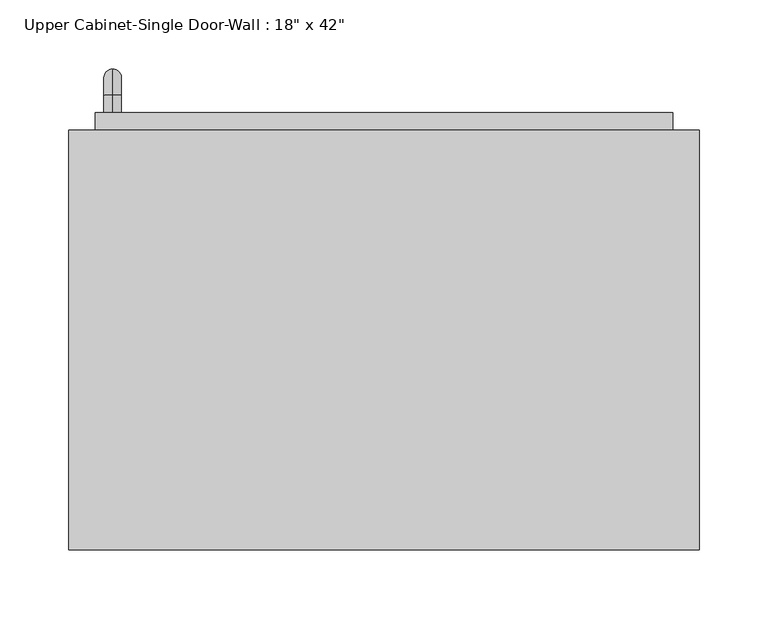
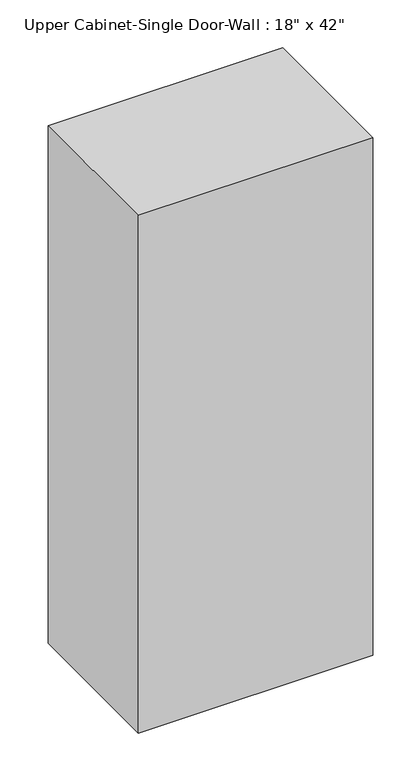
"""IFC4 building model written with IfcOpenShell, lengths in millimetres: furniture geometry."""

from ifc_helpers import new_model, si_unit, point, frame, origin, place, context, project, spatial, polyline, circle_curve, ellipse_curve, trimmed, outline, extrude, faceted_brep, source, transform, mapped, element, save
from ifc_brep_helpers import plane_surface, cylinder_surface, revolved_surface, advanced_brep


def furniture_a1406c10(model_context):
    return source(origin(), model_context, "Body", "SolidModel", [
        faceted_brep([(-198.8288372, 61.9125, 2438.4), (-198.8288372, 61.9125, 1371.6), (258.3711628, 61.9125, 1371.6), (258.3711628, 61.9125, 2438.4), (-198.8288372, 366.7125, 2438.4), (258.3711628, 366.7125, 2438.4), (258.3711628, 366.7125, 1371.6), (-198.8288372, 366.7125, 1371.6), (-179.7788372, 366.7125, 2419.35), (-179.7788372, 366.7125, 1390.65), (239.3211628, 366.7125, 1390.65), (239.3211628, 366.7125, 2419.35), (239.3211628, 80.9625, 2419.35), (-179.7788372, 80.9625, 2419.35), (239.3211628, 80.9625, 1390.65), (-179.7788372, 80.9625, 1390.65)], [[[0, 1, 2, 3]], [[4, 5, 6, 7], [8, 9, 10, 11]], [[1, 0, 4, 7]], [[2, 1, 7, 6]], [[3, 2, 6, 5]], [[0, 3, 5, 4]], [[8, 11, 12, 13]], [[11, 10, 14, 12]], [[10, 9, 15, 14]], [[9, 8, 13, 15]], [[13, 12, 14, 15]]]),
        advanced_brep(
        [(-167.0788372, 379.4125, 1517.65), (-167.0788372, 379.4125, 1530.35), (-167.0788372, 392.1125, 1517.65), (-167.0788372, 392.1125, 1530.35), (-167.0788372, 411.1625, 1511.3), (-167.0788372, 398.4625, 1511.3), (-167.0788372, 398.4625, 1435.1), (-167.0788372, 411.1625, 1435.1), (-167.0788372, 392.1125, 1416.05), (-167.0788372, 392.1125, 1428.75), (-167.0788372, 379.4125, 1428.75), (-167.0788372, 379.4125, 1416.05)],
        [
            (0, 1, circle_curve(frame((-167.0788372, 379.4125, 1524.0), z_axis=(0.0, -1.0, 0.0), x_axis=(0.0, 0.0, 1.0)), 6.35)),
            (1, 0, circle_curve(frame((-167.0788372, 379.4125, 1524.0), z_axis=(0.0, -1.0, 0.0), x_axis=(0.0, 0.0, 1.0)), 6.35)),
            (0, 2),
            (2, 3, circle_curve(frame((-167.0788372, 392.1125, 1524.0), z_axis=(0.0, -1.0, 0.0), x_axis=(0.0, 0.0, 1.0)), 6.35)),
            (3, 1),
            (3, 2, circle_curve(frame((-167.0788372, 392.1125, 1524.0), z_axis=(0.0, -1.0, 0.0), x_axis=(0.0, 0.0, 1.0)), 6.35)),
            (4, 3, circle_curve(frame((-167.0788372, 392.1125, 1511.3), z_axis=(1.0, 0.0, 0.0), x_axis=(0.0, 0.0, 1.0)), 19.05)),
            (2, 5, circle_curve(frame((-167.0788372, 392.1125, 1511.3), z_axis=(-1.0, 0.0, 0.0), x_axis=(0.0, 0.0, 1.0)), 6.35)),
            (5, 4, circle_curve(frame((-167.0788372, 404.8125, 1511.3), z_axis=(0.0, 0.0, 1.0), x_axis=(0.0, 1.0, 0.0)), 6.35)),
            (4, 5, circle_curve(frame((-167.0788372, 404.8125, 1511.3), z_axis=(0.0, 0.0, 1.0), x_axis=(0.0, 1.0, 0.0)), 6.35)),
            (5, 6),
            (6, 7, circle_curve(frame((-167.0788372, 404.8125, 1435.1), z_axis=(0.0, 0.0, 1.0), x_axis=(0.0, 1.0, 0.0)), 6.35)),
            (7, 4),
            (7, 6, circle_curve(frame((-167.0788372, 404.8125, 1435.1), z_axis=(0.0, 0.0, 1.0), x_axis=(0.0, 1.0, 0.0)), 6.35)),
            (8, 7, circle_curve(frame((-167.0788372, 392.1125, 1435.1), z_axis=(1.0, 0.0, 0.0), x_axis=(0.0, 1.0, 0.0)), 19.05)),
            (6, 9, circle_curve(frame((-167.0788372, 392.1125, 1435.1), z_axis=(-1.0, 0.0, 0.0), x_axis=(0.0, 1.0, 0.0)), 6.35)),
            (9, 8, circle_curve(frame((-167.0788372, 392.1125, 1422.4), z_axis=(0.0, 1.0, 0.0), x_axis=(0.0, 0.0, -1.0)), 6.35)),
            (8, 9, circle_curve(frame((-167.0788372, 392.1125, 1422.4), z_axis=(0.0, 1.0, 0.0), x_axis=(0.0, 0.0, -1.0)), 6.35)),
            (10, 11, circle_curve(frame((-167.0788372, 379.4125, 1422.4), z_axis=(0.0, -1.0, 0.0), x_axis=(0.0, 0.0, -1.0)), 6.35)),
            (11, 10, circle_curve(frame((-167.0788372, 379.4125, 1422.4), z_axis=(0.0, -1.0, 0.0), x_axis=(0.0, 0.0, -1.0)), 6.35)),
            (9, 10),
            (11, 8),
        ],
        [
            plane_surface(frame((-173.4288372, 379.4125, 1524.0), z_axis=(0.0, -1.0, 0.0), x_axis=(0.0, 0.0, 1.0))),
            cylinder_surface(frame((-167.0788372, 379.4125, 1524.0), z_axis=(0.0, -1.0, 0.0), x_axis=(0.0, 0.0, 1.0)), 6.35),
            revolved_surface(trimmed(ellipse_curve(frame((-167.0788372, 392.1125, 1524.0), z_axis=(0.0, -1.0, 0.0), x_axis=(0.0, 0.0, 1.0)), 6.35, 6.35), [point((-167.0788372, 392.1125, 1517.65))], [point((-167.0788372, 392.1125, 1530.35))], True, "CARTESIAN"), (-167.0788372, 392.1125, 1511.3), (-1.0, 0.0, 0.0)),
            revolved_surface(trimmed(ellipse_curve(frame((-167.0788372, 392.1125, 1524.0), z_axis=(0.0, -1.0, 0.0), x_axis=(0.0, 0.0, 1.0)), 6.35, 6.35), [point((-167.0788372, 392.1125, 1530.35))], [point((-167.0788372, 392.1125, 1517.65))], True, "CARTESIAN"), (-167.0788372, 392.1125, 1511.3), (-1.0, 0.0, 0.0)),
            cylinder_surface(frame((-167.0788372, 404.8125, 1511.3), z_axis=(0.0, 0.0, 1.0), x_axis=(0.0, 1.0, 0.0)), 6.35),
            revolved_surface(trimmed(ellipse_curve(frame((-167.0788372, 404.8125, 1435.1), z_axis=(0.0, 0.0, 1.0), x_axis=(0.0, 1.0, 0.0)), 6.35, 6.35), [point((-167.0788372, 398.4625, 1435.1))], [point((-167.0788372, 411.1625, 1435.1))], True, "CARTESIAN"), (-167.0788372, 392.1125, 1435.1), (-1.0, 0.0, 0.0)),
            revolved_surface(trimmed(ellipse_curve(frame((-167.0788372, 404.8125, 1435.1), z_axis=(0.0, 0.0, 1.0), x_axis=(0.0, 1.0, 0.0)), 6.35, 6.35), [point((-167.0788372, 411.1625, 1435.1))], [point((-167.0788372, 398.4625, 1435.1))], True, "CARTESIAN"), (-167.0788372, 392.1125, 1435.1), (-1.0, 0.0, 0.0)),
            plane_surface(frame((-173.4288372, 379.4125, 1422.4), z_axis=(0.0, -1.0, 0.0), x_axis=(0.0, 0.0, -1.0))),
            cylinder_surface(frame((-167.0788372, 392.1125, 1422.4), z_axis=(0.0, 1.0, 0.0), x_axis=(0.0, 0.0, -1.0)), 6.35),
        ],
        [
            (0, [[1, 2]]),
            (1, [[-1, 3, 4, 5]]),
            (1, [[-2, -5, 6, -3]]),
            (2, [[7, -4, 8, 9]]),
            (3, [[-8, -6, -7, 10]]),
            (4, [[-9, 11, 12, 13]]),
            (4, [[-10, -13, 14, -11]]),
            (5, [[15, -12, 16, 17]]),
            (6, [[-16, -14, -15, 18]]),
            (7, [[19, 20]]),
            (8, [[-17, 21, -20, 22]]),
            (8, [[-18, -22, -19, -21]]),
        ],
    ),
        extrude(outline(polyline([(-179.7788372, 379.4125), (239.3211628, 379.4125), (239.3211628, 347.6625), (-179.7788372, 347.6625), (-179.7788372, 379.4125)])), frame((0.0, 0.0, 1390.65), z_axis=(0.0, 0.0, 1.0), x_axis=(1.0, 0.0, 0.0)), (0.0, 0.0, 1.0), 1028.7),
    ])


if __name__ == "__main__":
    model = new_model("IFC4")
    model_context = context("Model", 3, world=origin())
    ifc_project = project(units=[si_unit("LENGTHUNIT", "METRE", prefix="MILLI")], contexts=[model_context])
    site = spatial("IfcSite", under=ifc_project)
    building = spatial("IfcBuilding", under=site)
    placement = place(None, origin())
    furniture_shape = furniture_a1406c10(model_context)
    element("IfcFurniture", 1, ObjectType="Upper Cabinet-Single Door-Wall : 18\" x 42\"", at=placement, inside=building, context=model_context, shape_type="MappedRepresentation", body=[
        mapped(furniture_shape, transform((0.0, 0.0, 0.0), x_axis=(1.0, 0.0, 0.0), y_axis=(0.0, 1.0, 0.0), z_axis=(0.0, 0.0, 1.0))),
    ])
    save(model, "model.ifc")

# Revit data of these elements
# Type "Upper Cabinet-Single Door-Wall : 18\" x 42\""
#   COBie.Type.CreatedBy = "doug.wood@us.ibm.com"
#   COBie.Type.CreatedOn = "2016-04-14T02:07:23"
#   COBie.Type.Name = "Casework_Upper Cabinet-Single Door-Wall_18\" x 42\""
#   COBie.Type.Category = "23-40 35 17 47 11 : Kitchen Casework"
#   COBie.Type.Description = "Upper Cabinet-Single Door-Wall_18\" x 42\""
#   COBie.Type.Manufacturer = ""
#   COBie.Type.ModelNumber = ""
#   Assembly Code = "C1030410"
#   COBie.Type.ReplacementCost = 0
#   Depth = 1' - 0"
#   Height = 3' - 6"
#   Top Of Cabinet = 8' - 0"
#   Width = 1' - 6"
#   COBie.Type = no
#   Cabinet Material = none
#   Door/Drawer Material = none
#   Handle Material = Cabinets - Handles
# Element 1 (IfcFurniture, "Upper Cabinet-Single Door-Wall : 18\" x 42\"")
#   Materials on its faces: "Cabinets", "Cabinets - Handles"
# Materials
#   "Cabinets - Handles": class "Metal", colour RGB 57 57 57, transparency 0
#   "Cabinets": class "Miscellaneous", colour RGB 249 249 249, transparency 0
